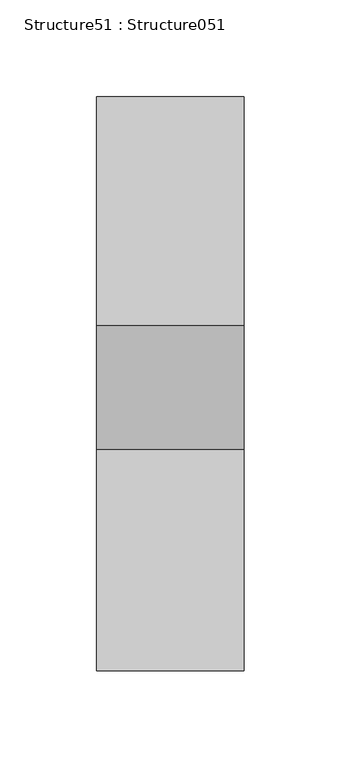
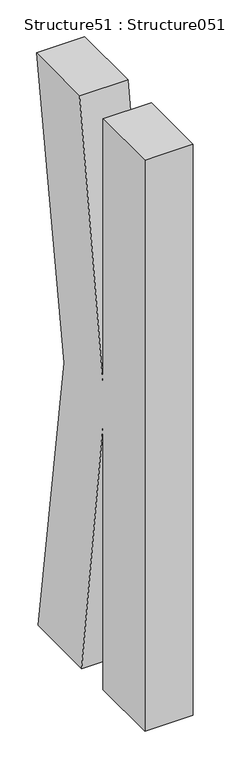
"""IFC4 building model written with IfcOpenShell, lengths in millimetres: proxy geometry, Structure51 : Structure051."""

from ifc_helpers import new_model, si_unit, frame, origin, place, context, project, spatial, polyline, outline, extrude, source, transform, mapped, element, save


def structure51_structure051_ac79a77f(model_context):
    return source(origin(), model_context, "Body", "SweptSolid", [
        extrude(outline(polyline([(250227.2968104, 3528.5825142), (250107.6375922, 3528.5825142), (250049.1720982, 3969.1658661), (250049.1720982, 3528.5825142), (249934.9277746, 3528.5825142), (249934.9277746, 4480.4419946), (250049.1720982, 4480.4419946), (250049.1720982, 4038.5077532), (250113.0783079, 4480.4419946), (250231.3815982, 4480.4419946), (250155.221025, 4009.9589531), (250227.2968104, 3528.5825142)])), frame((-38594.2176606, 0.0, 0.0), z_axis=(1.0, 0.0, 0.0), x_axis=(0.0, 1.0, 0.0)), (0.0, 0.0, 1.0), 76.2),
    ])


if __name__ == "__main__":
    model = new_model("IFC4")
    model_context = context("Model", 3, world=origin())
    ifc_project = project(units=[si_unit("LENGTHUNIT", "METRE", prefix="MILLI")], contexts=[model_context])
    site = spatial("IfcSite", under=ifc_project)
    building = spatial("IfcBuilding", under=site)
    placement = place(None, origin())
    structure51_structure051_shape = structure51_structure051_ac79a77f(model_context)
    element("IfcBuildingElementProxy", 1, Name="Structure51 : Structure051", ObjectType="Structure51 : Structure051", at=placement, inside=building, context=model_context, shape_type="MappedRepresentation", body=[
        mapped(structure51_structure051_shape, transform((0.0, 0.0, 0.0), x_axis=(1.0, 0.0, 0.0), y_axis=(0.0, 1.0, 0.0), z_axis=(0.0, 0.0, 1.0))),
    ])
    save(model, "model.ifc")

# Revit data of these elements
# Type "Structure51 : Structure051"
#   NameOverride = "Structure051"
# Element 1 (IfcBuildingElementProxy, "Structure51 : Structure051")
#   Materials on its faces: "BRUSHED ALUM. LETTERING"
# Materials
#   "BRUSHED ALUM. LETTERING": class "Unassigned", colour RGB 169 181 186, transparency 0, Cost = 0
